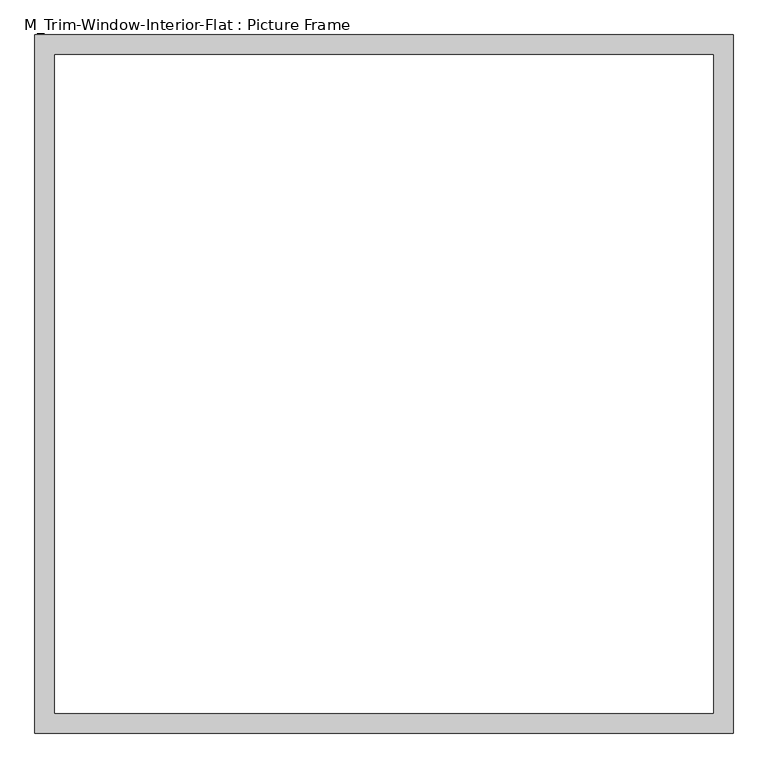
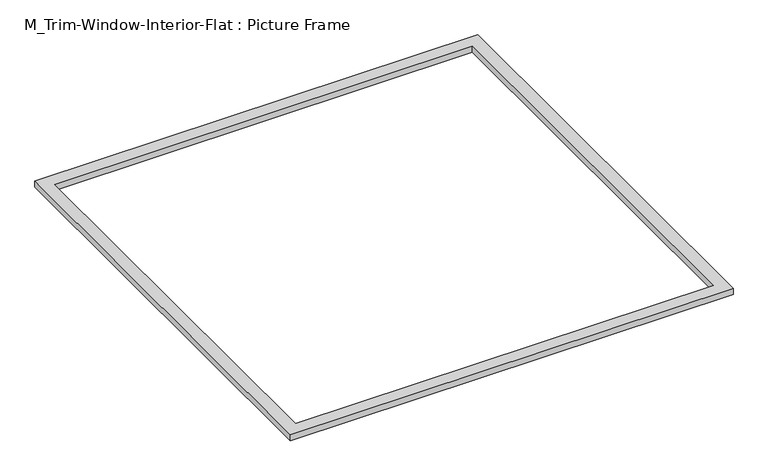
"""IFC4 building model written with IfcOpenShell, lengths in millimetres: proxy geometry, M_Trim-Window-Interior-Flat : Picture Frame."""

from ifc_helpers import new_model, si_unit, origin, origin_with_axes, place, context, project, spatial, polyline, outline, extrude, source, transform, mapped, element, save


def m_trim_window_interior_flat_picture_frame_b3916ce1(model_context):
    return source(origin(), model_context, "Body", "SweptSolid", [
        extrude(outline(polyline([(1047.3, 47.3), (1047.3, -2047.3), (-1047.3, -2047.3), (-1047.3, 47.3), (1047.3, 47.3)]), holes=[polyline([(987.3, -12.7), (-987.3, -12.7), (-987.3, -1987.3), (987.3, -1987.3), (987.3, -12.7)])]), origin_with_axes(), (0.0, 0.0, 1.0), 30.0),
    ])


if __name__ == "__main__":
    model = new_model("IFC4")
    model_context = context("Model", 3, world=origin())
    ifc_project = project(units=[si_unit("LENGTHUNIT", "METRE", prefix="MILLI")], contexts=[model_context])
    site = spatial("IfcSite", under=ifc_project)
    building = spatial("IfcBuilding", under=site)
    placement = place(None, origin())
    m_trim_window_interior_flat_picture_frame_shape = m_trim_window_interior_flat_picture_frame_b3916ce1(model_context)
    element("IfcBuildingElementProxy", 1, Name="M_Trim-Window-Interior-Flat : Picture Frame", ObjectType="M_Trim-Window-Interior-Flat : Picture Frame", at=placement, inside=building, context=model_context, shape_type="MappedRepresentation", body=[
        mapped(m_trim_window_interior_flat_picture_frame_shape, transform((0.0, 0.0, 0.0), x_axis=(1.0, 0.0, 0.0), y_axis=(0.0, 1.0, 0.0), z_axis=(0.0, 0.0, 1.0))),
    ])
    save(model, "model.ifc")

# Revit data of these elements
# Type "M_Trim-Window-Interior-Flat : Picture Frame"
#   Trim Thickness_Picture Frame = 30 mm
#   Trim Width = 60 mm
#   Trim Thickness_with Sill = 20 mm
#   Sill Thickness = 30 mm
#   Opening Width [instance default] = 600 mm
#   Opening Height [instance default] = 900 mm
#   Default Elevation = 1200 mm
#   Sill = no
#   Picture Frame = yes
#   Trim Material [instance default] = none
# Element 1 (IfcBuildingElementProxy, "M_Trim-Window-Interior-Flat : Picture Frame")
#   Opening Width = 2000 mm
#   Opening Height = 2000 mm
#   Trim Material = Wood - Stained
#   Materials on its faces: "Wood - Stained"
# Materials
#   "Wood - Stained": class "Wood", colour RGB 173 132 96, transparency 0, Cost = 0
